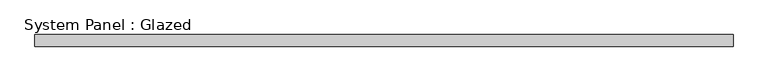
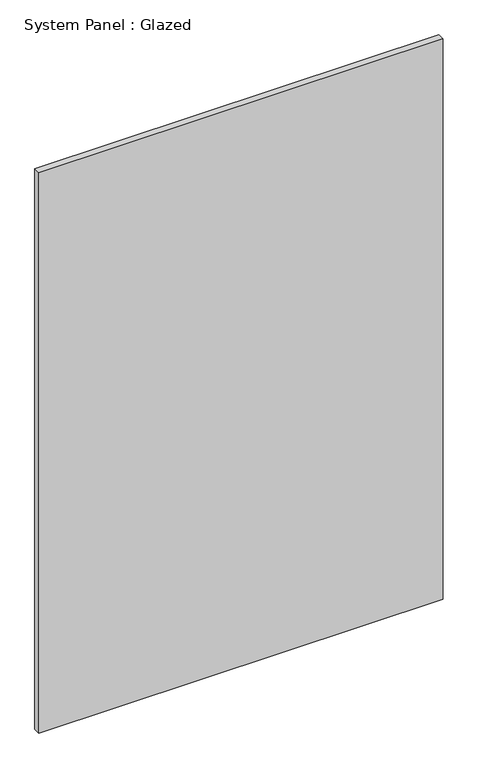
"""IFC4 building model written with IfcOpenShell, lengths in millimetres: plate geometry, System Panel : Glazed."""

from ifc_helpers import new_model, si_unit, origin, origin_with_axes, place, context, project, spatial, polyline, outline, extrude, source, transform, mapped, element, save


def system_panel_glazed_c51f38ac(model_context):
    return source(origin(), model_context, "Body", "SweptSolid", [
        extrude(outline(polyline([(725.0514967, -49.5), (-725.0514967, -49.5), (-725.0514967, -24.5), (725.0514967, -24.5), (725.0514967, -49.5)])), origin_with_axes(), (0.0, 0.0, 1.0), 2125.0),
    ])


if __name__ == "__main__":
    model = new_model("IFC4")
    model_context = context("Model", 3, world=origin())
    ifc_project = project(units=[si_unit("LENGTHUNIT", "METRE", prefix="MILLI")], contexts=[model_context])
    site = spatial("IfcSite", under=ifc_project)
    building = spatial("IfcBuilding", under=site)
    placement = place(None, origin())
    system_panel_glazed_shape = system_panel_glazed_c51f38ac(model_context)
    element("IfcPlate", 1, ObjectType="System Panel : Glazed", at=placement, inside=building, context=model_context, shape_type="MappedRepresentation", body=[
        mapped(system_panel_glazed_shape, transform((0.0, 0.0, 0.0), x_axis=(1.0, 0.0, 0.0), y_axis=(0.0, 1.0, 0.0), z_axis=(0.0, 0.0, 1.0))),
    ])
    save(model, "model.ifc")

# Revit data of these elements
# Type "System Panel : Glazed"
#   Keynote = "H11"
#   Construction Type Id = "GSP4R"
#   Analytic Construction = "1/8 in Pilkington single glazing"
#   Visual Light Transmittance = 0.9
#   Solar Heat Gain Coefficient = 0.86
#   Heat Transfer Coefficient (U) = 6.7069 W/(m²·K)
# Element 1 (IfcPlate, "System Panel : Glazed")
#   Materials on its faces: "Glass"
# Materials
#   "Glass": class "Glass", colour RGB 0 128 192, transparency 0.9, Description = "Soda Lime Glass", Cost = 0
